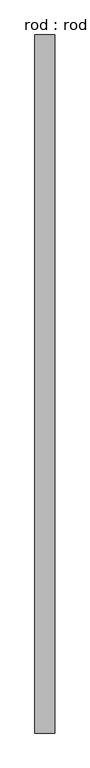
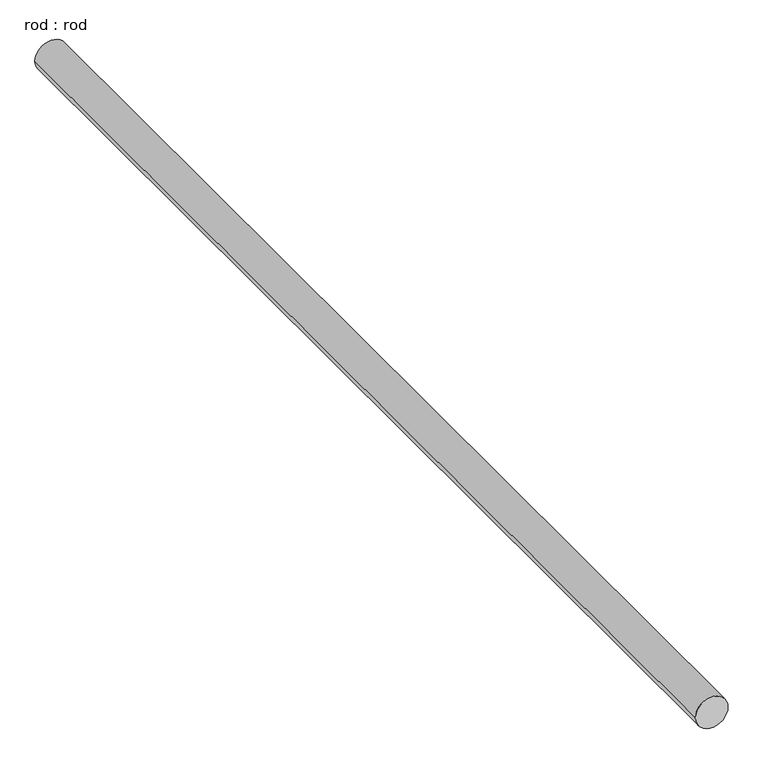
"""IFC4 building model written with IfcOpenShell, lengths in millimetres: proxy geometry, rod : rod."""

from ifc_helpers import new_model, si_unit, point, frame, frame_2d, origin, place, context, project, spatial, circle_curve, trimmed, segment, composite_curve, outline, extrude, source, transform, mapped, element, save


def rod_rod_1436e789(model_context):
    return source(origin(), model_context, "Body", "SweptSolid", [
        extrude(outline(composite_curve([segment(trimmed(circle_curve(frame_2d((0.0108462, 0.0)), 200.0), [point((0.0108462, 200.0))], [point((0.0108462, -200.0))], False, "CARTESIAN"), True, "CONTINUOUS"), segment(trimmed(circle_curve(frame_2d((0.0108462, 0.0)), 200.0), [point((0.0108462, -200.0))], [point((0.0108462, 200.0))], False, "CARTESIAN"), True, "CONTINUOUS")], self_intersect=False)), frame((0.0, -2938.9540947, 0.0), z_axis=(0.0, 1.0, 0.0), x_axis=(0.0, 0.0, 1.0)), (0.0, 0.0, 1.0), 14063.3654201),
    ])


if __name__ == "__main__":
    model = new_model("IFC4")
    model_context = context("Model", 3, world=origin())
    ifc_project = project(units=[si_unit("LENGTHUNIT", "METRE", prefix="MILLI")], contexts=[model_context])
    site = spatial("IfcSite", under=ifc_project)
    building = spatial("IfcBuilding", under=site)
    placement = place(None, origin())
    rod_rod_shape = rod_rod_1436e789(model_context)
    element("IfcBuildingElementProxy", 1, Name="rod : rod", ObjectType="rod : rod", at=placement, inside=building, context=model_context, shape_type="MappedRepresentation", body=[
        mapped(rod_rod_shape, transform((0.0, 0.0, 0.0), x_axis=(1.0, 0.0, 0.0), y_axis=(0.0, 1.0, 0.0), z_axis=(0.0, 0.0, 1.0))),
    ])
    save(model, "model.ifc")

# Revit data of these elements
# Type "rod : rod"
#   Default Elevation = 0
